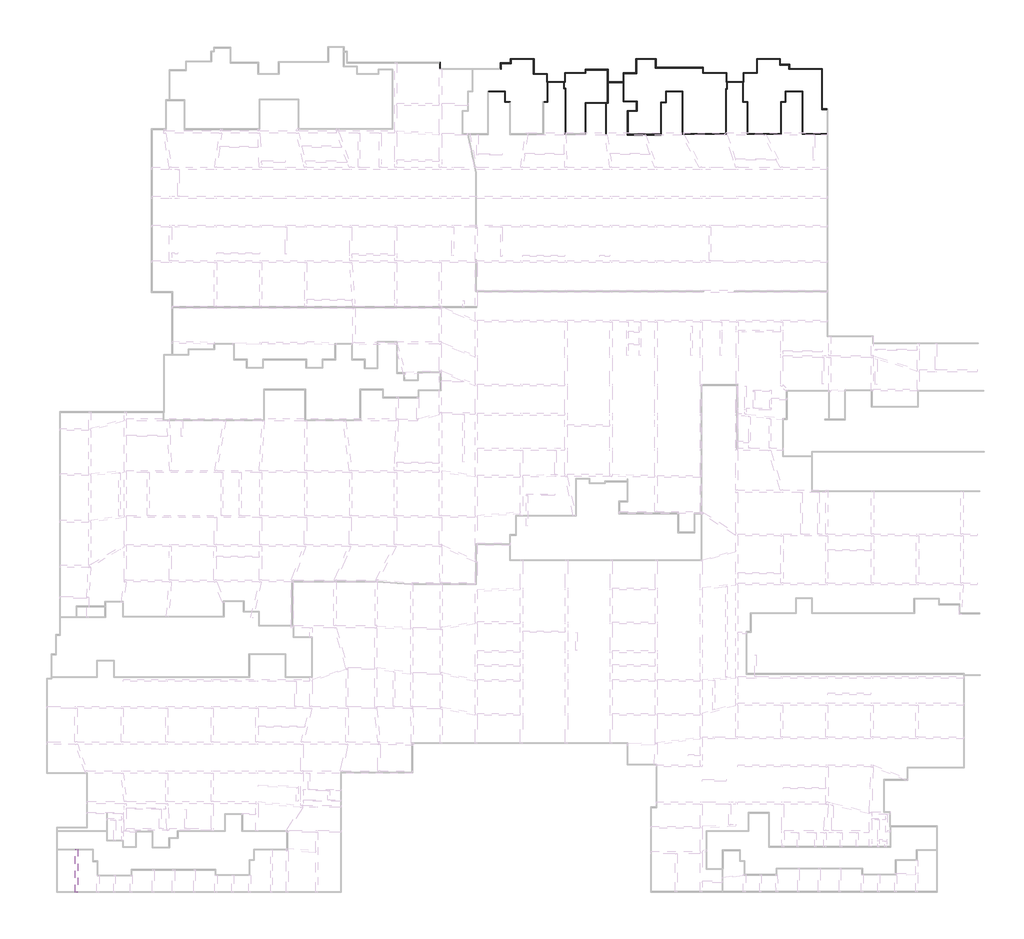
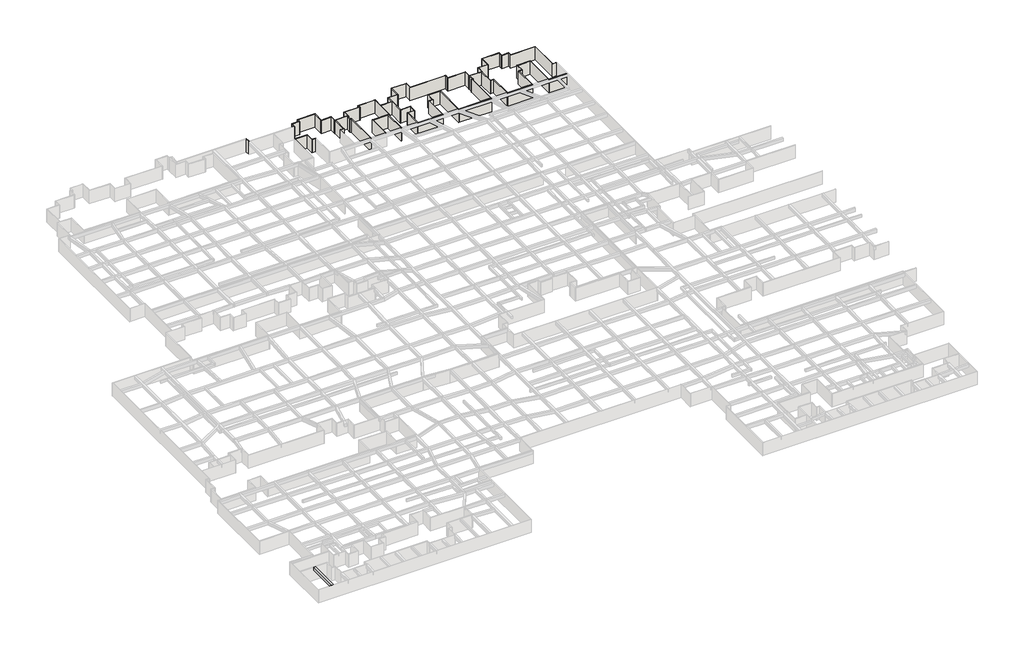
# One storey, part 5 of 16: 70 walls, 1 beam.
# Revit data of these elements (continued)
# Type "混凝土 - 矩形梁 : KL_beam"
#   Length [instance default] = 1524 mm
#   b = 400 mm
#   h = 800 mm
#   Structural Material [instance default] = 混凝土 - 现场浇注混凝土
#   Assembly Code = ""
# Type "所有墙体"
#   Layers, outside or top first: 120 mm "默认" (function 1)
# Element 1 (IfcBeam, "混凝土 - 矩形梁 : KL_beam")
#   Comments = ""
#   Structural Material = none
#   Phase Created = 新构造
# Elements 2, 3, 4, 5, 6, 7, 8, 9, 10, 11, 12, 13, 14, 15, 16, 17, 18, 19, 20, 21, 22, 23, 24, 25, 26, 27, 28, 29, 30, 31, 32, 33, 34, 35, 36, 37, 38, 39, 40, 41, 42, 43, 44, 45, 46, 47, 48, 49, 50, 51, 52, 53, 54, 55, 56, 57, 58, 59, 60, 61, 62, 63, 64, 65, 66, 67, 68, 69, 70, 71 (IfcWall, "所有墙体")
#   Top Offset = 0 mm
#   Base Offset = 0 mm
#   wall height = 3300 mm
#   Phase Created = 新构造
#   Base Constraint = 户型图
#   Top Constraint = 层高
#   Materials on its faces: "默认"
# Materials
#   "混凝土 - 现场浇注混凝土": class "混凝土", colour RGB 192 192 192, transparency 0
#   "默认": class "其他", colour RGB 192 192 192, transparency 0, Cost = 0
